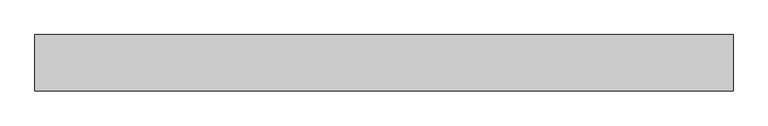
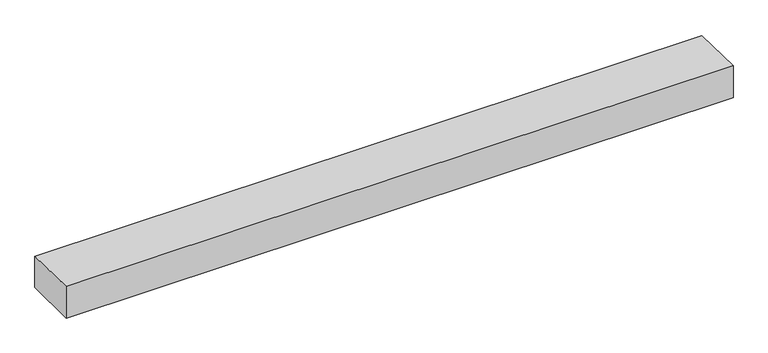
"""IFC4 building model written with IfcOpenShell, lengths in millimetres: proxy geometry, Generic Models 7:Generic Models 1:6:Generic Models 1:6 : Generic Models 7:Generic Models 1:337419:8 : Generic Models 7:Generic Models 1:6:Generic Models 1:6 : Generic Models 7:Generic Models 1:337419:312901."""

from ifc_helpers import new_model, si_unit, frame, origin, place, context, project, spatial, polyline, outline, extrude, source, transform, mapped, element, save


def generic_models_8530d58a(model_context):
    return source(origin(), model_context, "Body", "SweptSolid", [
        extrude(outline(polyline([(-536354.0913358, -4.2333333), (-536354.0913358, -127.0), (-536557.2913358, -127.0), (-536557.2913358, 0.0), (-536354.0913358, -4.2333333)])), frame((591306.0367242, 0.0, 0.0), z_axis=(1.0, 0.0, 0.0), x_axis=(0.0, 1.0, 0.0)), (0.0, 0.0, 1.0), 2515.1138527),
    ])


if __name__ == "__main__":
    model = new_model("IFC4")
    model_context = context("Model", 3, world=origin())
    ifc_project = project(units=[si_unit("LENGTHUNIT", "METRE", prefix="MILLI")], contexts=[model_context])
    site = spatial("IfcSite", under=ifc_project)
    building = spatial("IfcBuilding", under=site)
    placement = place(None, origin())
    generic_models_shape = generic_models_8530d58a(model_context)
    element("IfcBuildingElementProxy", 1, Name="Generic Models 7:Generic Models 1:6:Generic Models 1:6 : Generic Models 7:Generic Models 1:337419:8 : Generic Models 7:Generic Models 1:6:Generic Models 1:6 : Generic Models 7:Generic Models 1:337419:312901", ObjectType="Generic Models 7:Generic Models 1:6:Generic Models 1:6 : Generic Models 7:Generic Models 1:337419:8 : Generic Models 7:Generic Models 1:6:Generic Models 1:6 : Generic Models 7:Generic Models 1:337419:312901", at=placement, inside=building, context=model_context, shape_type="MappedRepresentation", body=[
        mapped(generic_models_shape, transform((0.0, 0.0, 0.0), x_axis=(1.0, 0.0, 0.0), y_axis=(0.0, 1.0, 0.0), z_axis=(0.0, 0.0, 1.0))),
    ])
    save(model, "model.ifc")

# Revit data of these elements
# Type "Generic Models 7:Generic Models 1:6:Generic Models 1:6 : Generic Models 7:Generic Models 1:337419:8 : Generic Models 7:Generic Models 1:6:Generic Models 1:6 : Generic Models 7:Generic Models 1:337419:312901"
#   NameOverride = "Generic Models 7:Generic Models 1:6:Generic Models 1:6 : Generic Models 7:Generic Models 1:337419:312901"
#   ObjectTypeOverride = "Generic Models 1:6 : Generic Models 7:Generic Models 1:337419"
#   Reference = "Generic Models 1"
#   Tag = "312901"
# Element 1 (IfcBuildingElementProxy, "Generic Models 7:Generic Models 1:6:Generic Models 1:6 : Generic Models 7:Generic Models 1:337419:8 : Generic Models 7:Generic Models 1:6:Generic Models 1:6 : Generic Models 7:Generic Models 1:337419:312901")
#   Materials on its faces: "CONCRETE PAVEMENT/SIDEWALK - SLOPE (2%) AWAY BUILDING"
# Materials
#   "CONCRETE PAVEMENT/SIDEWALK - SLOPE (2%) AWAY BUILDING": class "Concrete", colour RGB 115 116 108, transparency 0, Description = "Lightweight concrete", Cost = 0
